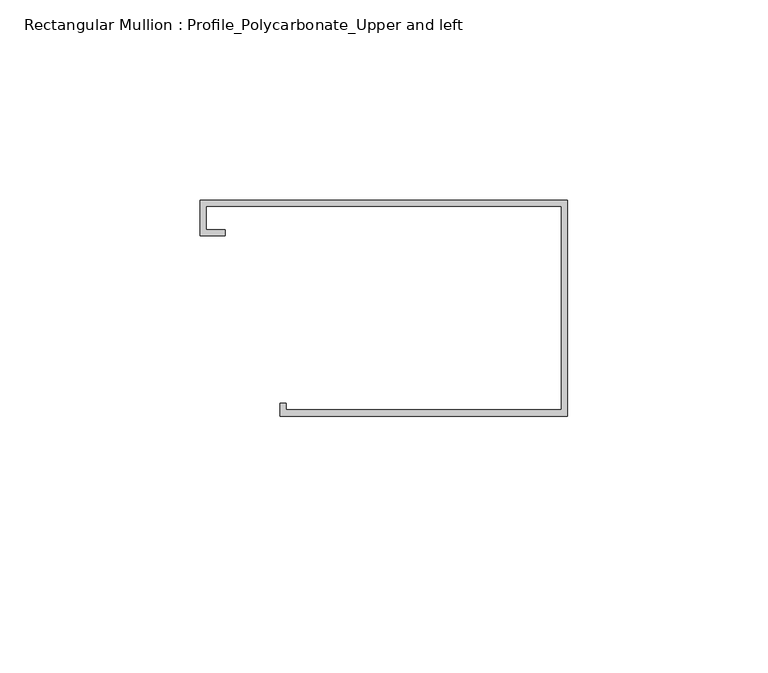
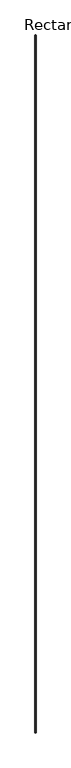
"""IFC4 building model written with IfcOpenShell, lengths in millimetres: member geometry, Rectangular Mullion : Profile_Polycarbonate_Upper and left."""

from ifc_helpers import new_model, si_unit, frame, origin, place, context, project, spatial, polyline, outline, extrude, source, transform, mapped, element, save


def rectangular_mullion_profile_polycarbonate_upper_and_left_5675727e(model_context):
    return source(origin(), model_context, "Body", "SweptSolid", [
        extrude(outline(polyline([(0.0, 28.984575), (0.0, -25.015825), (-71.9836, -25.015825), (-71.9836, -21.840825), (-70.3961, -21.840825), (-70.3961, -23.428325), (-1.5875, -23.428325), (-1.5875, 27.397075), (-90.4113, 27.397075), (-90.4113, 21.580475), (-85.6488, 21.580475), (-85.6488, 19.992975), (-91.9988, 19.992975), (-91.9988, 28.984575), (0.0, 28.984575)])), frame((0.0, 0.0, -80941.7668531), z_axis=(0.0, 0.0, 1.0), x_axis=(1.0, 0.0, 0.0)), (0.0, 0.0, 1.0), 80941.7668531),
    ])


if __name__ == "__main__":
    model = new_model("IFC4")
    model_context = context("Model", 3, world=origin())
    ifc_project = project(units=[si_unit("LENGTHUNIT", "METRE", prefix="MILLI")], contexts=[model_context])
    site = spatial("IfcSite", under=ifc_project)
    building = spatial("IfcBuilding", under=site)
    placement = place(None, origin())
    rectangular_mullion_profile_polycarbonate_upper_and_left_shape = rectangular_mullion_profile_polycarbonate_upper_and_left_5675727e(model_context)
    element("IfcMember", 1, ObjectType="Rectangular Mullion : Profile_Polycarbonate_Upper and left", at=placement, inside=building, context=model_context, shape_type="MappedRepresentation", body=[
        mapped(rectangular_mullion_profile_polycarbonate_upper_and_left_shape, transform((0.0, 0.0, 0.0), x_axis=(1.0, 0.0, 0.0), y_axis=(0.0, 1.0, 0.0), z_axis=(0.0, 0.0, 1.0))),
    ])
    save(model, "model.ifc")

# Revit data of these elements
# Type "Rectangular Mullion : Profile_Polycarbonate_Upper and left"
#   built-in parameter 1007322 = 0.177167 (stored number, unit not read)
#   built-in parameter 1007321 = 0.00520833 (stored number, unit not read)
#   built-in parameter 1007320 = 0 (stored number, unit not read)
